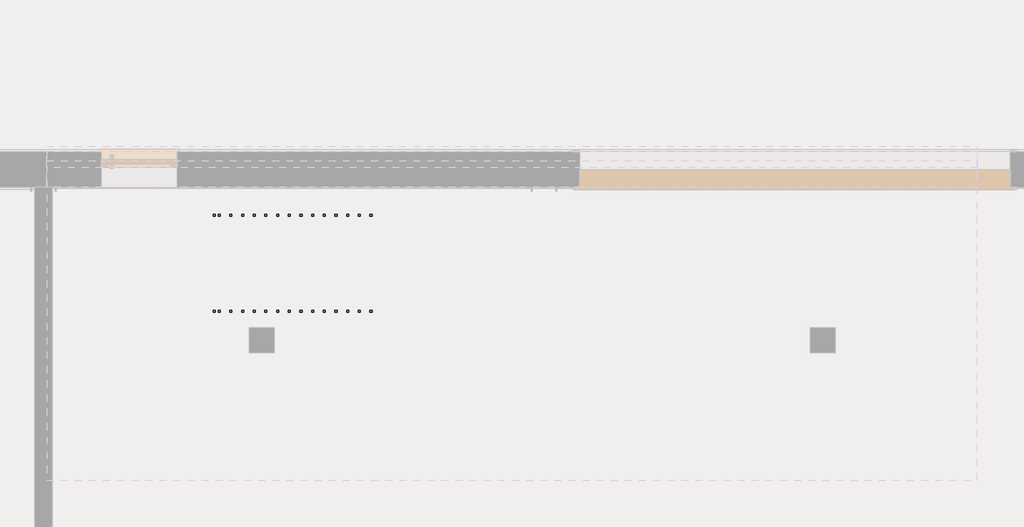
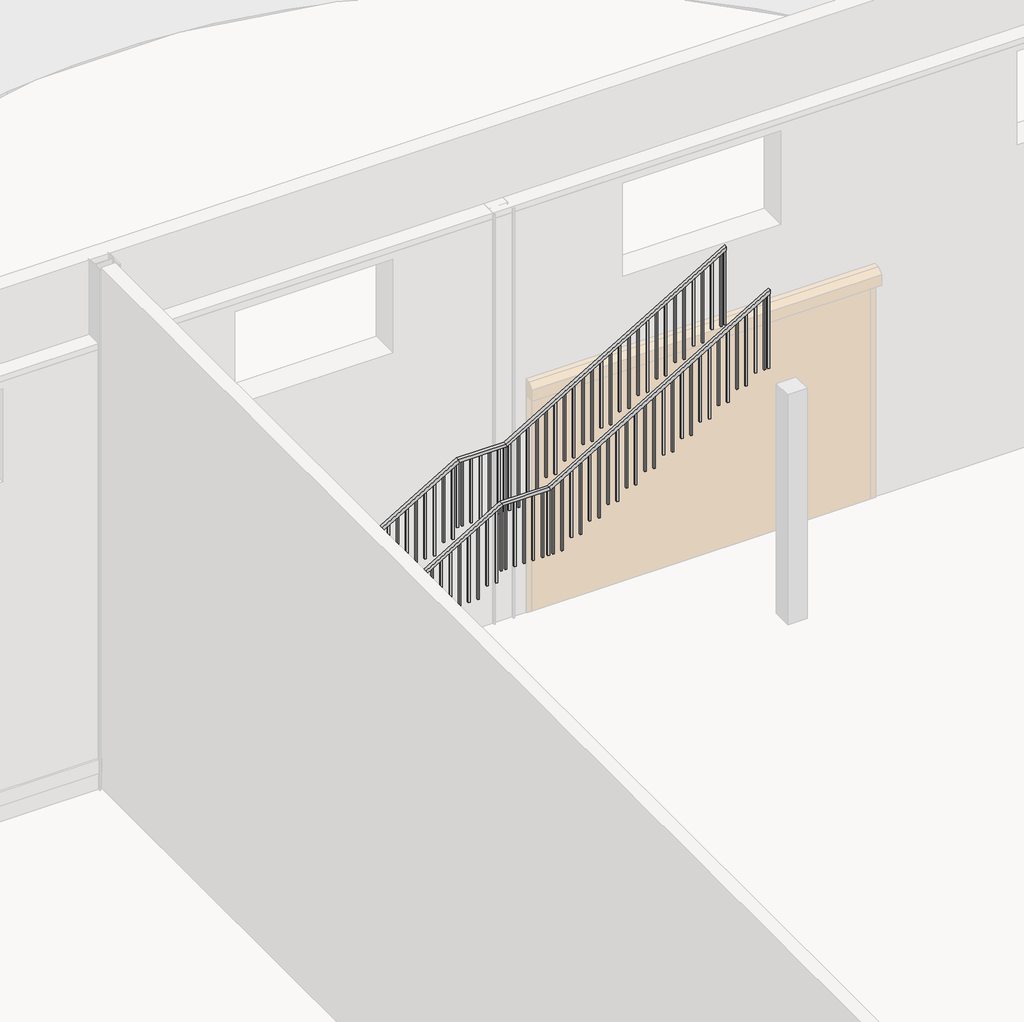
# One storey, part 11 of 13: 2 railings.
"""IFC4 building model written with IfcOpenShell, lengths in millimetres."""

from ifc_helpers import new_model, si_unit, frame, origin, place, context, project, spatial, polyline, outline, extrude, faceted_brep, element, save

model = new_model("IFC4")

# Units and contexts
model_context = context("Model", 3, world=origin())
ifc_project = project(units=[si_unit("LENGTHUNIT", "METRE", prefix="MILLI")], contexts=[model_context])

# Site, building, storey
site = spatial("IfcSite", under=ifc_project)
building = spatial("IfcBuilding", under=site)
storey = spatial("IfcBuildingStorey", under=building, Name="L0 - Ground Floor (Shadows On)", Elevation=0.0)

# Railings
placement = place(None, origin())
element("IfcRailing", 1, ObjectType="1100mm", at=placement, inside=storey, context=model_context, shape_type="SolidModel", body=[
    faceted_brep([(12896.9831159, 5374.1380918, 1266.6666667), (12896.9831159, 5374.1380918, 1208.4792885), (12896.9831159, 5324.1380918, 1208.4792885), (12896.9831159, 5324.1380918, 1266.6666667), (15976.9831159, 5374.1380918, 3100.0), (15990.7379111, 5374.1380918, 3050.0), (15990.7379111, 5324.1380918, 3050.0), (15976.9831159, 5324.1380918, 3100.0), (16696.9831159, 5374.1380918, 3100.0), (16710.7379111, 5374.1380918, 3050.0), (16710.7379111, 5324.1380918, 3050.0), (16696.9831159, 5324.1380918, 3100.0), (20056.9831159, 5374.1380918, 5100.0), (20056.9831159, 5324.1380918, 5100.0), (20056.9831159, 5324.1380918, 5041.8126219), (20056.9831159, 5374.1380918, 5041.8126219)], [[[0, 1, 2, 3]], [[1, 0, 4, 5]], [[2, 1, 5, 6]], [[3, 2, 6, 7]], [[0, 3, 7, 4]], [[5, 4, 8, 9]], [[6, 5, 9, 10]], [[7, 6, 10, 11]], [[4, 7, 11, 8]], [[12, 13, 14, 15]], [[9, 8, 12, 15]], [[10, 9, 15, 14]], [[11, 10, 14, 13]], [[8, 11, 13, 12]]]),
    extrude(outline(polyline([(4992.705479, 19974.4831159), (3833.3333333, 19974.4831159), (3833.3333333, 19999.4831159), (5007.5864314, 19999.4831159), (4992.705479, 19974.4831159)])), frame((0.0, 5336.6380918, 0.0), z_axis=(0.0, 1.0, 0.0), x_axis=(0.0, 0.0, 1.0)), (0.0, 0.0, 1.0), 25.0),
    extrude(outline(polyline([(4909.3721457, 19834.4831159), (3833.3333333, 19834.4831159), (3833.3333333, 19859.4831159), (4924.253098, 19859.4831159), (4909.3721457, 19834.4831159)])), frame((0.0, 5336.6380918, 0.0), z_axis=(0.0, 1.0, 0.0), x_axis=(0.0, 0.0, 1.0)), (0.0, 0.0, 1.0), 25.0),
    extrude(outline(polyline([(4826.0388123, 19694.4831159), (3666.6666667, 19694.4831159), (3666.6666667, 19719.4831159), (4840.9197647, 19719.4831159), (4826.0388123, 19694.4831159)])), frame((0.0, 5336.6380918, 0.0), z_axis=(0.0, 1.0, 0.0), x_axis=(0.0, 0.0, 1.0)), (0.0, 0.0, 1.0), 25.0),
    extrude(outline(polyline([(4742.705479, 19554.4831159), (3666.6666667, 19554.4831159), (3666.6666667, 19579.4831159), (4757.5864314, 19579.4831159), (4742.705479, 19554.4831159)])), frame((0.0, 5336.6380918, 0.0), z_axis=(0.0, 1.0, 0.0), x_axis=(0.0, 0.0, 1.0)), (0.0, 0.0, 1.0), 25.0),
    extrude(outline(polyline([(4659.3721457, 19414.4831159), (3500.0, 19414.4831159), (3500.0, 19439.4831159), (4674.253098, 19439.4831159), (4659.3721457, 19414.4831159)])), frame((0.0, 5336.6380918, 0.0), z_axis=(0.0, 1.0, 0.0), x_axis=(0.0, 0.0, 1.0)), (0.0, 0.0, 1.0), 25.0),
    extrude(outline(polyline([(4576.0388123, 19274.4831159), (3500.0, 19274.4831159), (3500.0, 19299.4831159), (4590.9197647, 19299.4831159), (4576.0388123, 19274.4831159)])), frame((0.0, 5336.6380918, 0.0), z_axis=(0.0, 1.0, 0.0), x_axis=(0.0, 0.0, 1.0)), (0.0, 0.0, 1.0), 25.0),
    extrude(outline(polyline([(4492.705479, 19134.4831159), (3333.3333333, 19134.4831159), (3333.3333333, 19159.4831159), (4507.5864314, 19159.4831159), (4492.705479, 19134.4831159)])), frame((0.0, 5336.6380918, 0.0), z_axis=(0.0, 1.0, 0.0), x_axis=(0.0, 0.0, 1.0)), (0.0, 0.0, 1.0), 25.0),
    extrude(outline(polyline([(4409.3721457, 18994.4831159), (3333.3333333, 18994.4831159), (3333.3333333, 19019.4831159), (4424.253098, 19019.4831159), (4409.3721457, 18994.4831159)])), frame((0.0, 5336.6380918, 0.0), z_axis=(0.0, 1.0, 0.0), x_axis=(0.0, 0.0, 1.0)), (0.0, 0.0, 1.0), 25.0),
    extrude(outline(polyline([(4326.0388123, 18854.4831159), (3166.6666667, 18854.4831159), (3166.6666667, 18879.4831159), (4340.9197647, 18879.4831159), (4326.0388123, 18854.4831159)])), frame((0.0, 5336.6380918, 0.0), z_axis=(0.0, 1.0, 0.0), x_axis=(0.0, 0.0, 1.0)), (0.0, 0.0, 1.0), 25.0),
    extrude(outline(polyline([(4242.705479, 18714.4831159), (3166.6666667, 18714.4831159), (3166.6666667, 18739.4831159), (4257.5864314, 18739.4831159), (4242.705479, 18714.4831159)])), frame((0.0, 5336.6380918, 0.0), z_axis=(0.0, 1.0, 0.0), x_axis=(0.0, 0.0, 1.0)), (0.0, 0.0, 1.0), 25.0),
    extrude(outline(polyline([(4159.3721457, 18574.4831159), (3000.0, 18574.4831159), (3000.0, 18599.4831159), (4174.253098, 18599.4831159), (4159.3721457, 18574.4831159)])), frame((0.0, 5336.6380918, 0.0), z_axis=(0.0, 1.0, 0.0), x_axis=(0.0, 0.0, 1.0)), (0.0, 0.0, 1.0), 25.0),
    extrude(outline(polyline([(4076.0388123, 18434.4831159), (3000.0, 18434.4831159), (3000.0, 18459.4831159), (4090.9197647, 18459.4831159), (4076.0388123, 18434.4831159)])), frame((0.0, 5336.6380918, 0.0), z_axis=(0.0, 1.0, 0.0), x_axis=(0.0, 0.0, 1.0)), (0.0, 0.0, 1.0), 25.0),
    extrude(outline(polyline([(3992.705479, 18294.4831159), (2833.3333333, 18294.4831159), (2833.3333333, 18319.4831159), (4007.5864314, 18319.4831159), (3992.705479, 18294.4831159)])), frame((0.0, 5336.6380918, 0.0), z_axis=(0.0, 1.0, 0.0), x_axis=(0.0, 0.0, 1.0)), (0.0, 0.0, 1.0), 25.0),
    extrude(outline(polyline([(3909.3721457, 18154.4831159), (2833.3333333, 18154.4831159), (2833.3333333, 18179.4831159), (3924.253098, 18179.4831159), (3909.3721457, 18154.4831159)])), frame((0.0, 5336.6380918, 0.0), z_axis=(0.0, 1.0, 0.0), x_axis=(0.0, 0.0, 1.0)), (0.0, 0.0, 1.0), 25.0),
    extrude(outline(polyline([(3826.0388123, 18014.4831159), (2666.6666667, 18014.4831159), (2666.6666667, 18039.4831159), (3840.9197647, 18039.4831159), (3826.0388123, 18014.4831159)])), frame((0.0, 5336.6380918, 0.0), z_axis=(0.0, 1.0, 0.0), x_axis=(0.0, 0.0, 1.0)), (0.0, 0.0, 1.0), 25.0),
    extrude(outline(polyline([(3742.705479, 17874.4831159), (2666.6666667, 17874.4831159), (2666.6666667, 17899.4831159), (3757.5864314, 17899.4831159), (3742.705479, 17874.4831159)])), frame((0.0, 5336.6380918, 0.0), z_axis=(0.0, 1.0, 0.0), x_axis=(0.0, 0.0, 1.0)), (0.0, 0.0, 1.0), 25.0),
    extrude(outline(polyline([(3659.3721457, 17734.4831159), (2500.0, 17734.4831159), (2500.0, 17759.4831159), (3674.253098, 17759.4831159), (3659.3721457, 17734.4831159)])), frame((0.0, 5336.6380918, 0.0), z_axis=(0.0, 1.0, 0.0), x_axis=(0.0, 0.0, 1.0)), (0.0, 0.0, 1.0), 25.0),
    extrude(outline(polyline([(3576.0388123, 17594.4831159), (2500.0, 17594.4831159), (2500.0, 17619.4831159), (3590.9197647, 17619.4831159), (3576.0388123, 17594.4831159)])), frame((0.0, 5336.6380918, 0.0), z_axis=(0.0, 1.0, 0.0), x_axis=(0.0, 0.0, 1.0)), (0.0, 0.0, 1.0), 25.0),
    extrude(outline(polyline([(3492.705479, 17454.4831159), (2333.3333333, 17454.4831159), (2333.3333333, 17479.4831159), (3507.5864314, 17479.4831159), (3492.705479, 17454.4831159)])), frame((0.0, 5336.6380918, 0.0), z_axis=(0.0, 1.0, 0.0), x_axis=(0.0, 0.0, 1.0)), (0.0, 0.0, 1.0), 25.0),
    extrude(outline(polyline([(3409.3721457, 17314.4831159), (2333.3333333, 17314.4831159), (2333.3333333, 17339.4831159), (3424.253098, 17339.4831159), (3409.3721457, 17314.4831159)])), frame((0.0, 5336.6380918, 0.0), z_axis=(0.0, 1.0, 0.0), x_axis=(0.0, 0.0, 1.0)), (0.0, 0.0, 1.0), 25.0),
    extrude(outline(polyline([(3326.0388123, 17174.4831159), (2166.6666667, 17174.4831159), (2166.6666667, 17199.4831159), (3340.9197647, 17199.4831159), (3326.0388123, 17174.4831159)])), frame((0.0, 5336.6380918, 0.0), z_axis=(0.0, 1.0, 0.0), x_axis=(0.0, 0.0, 1.0)), (0.0, 0.0, 1.0), 25.0),
    extrude(outline(polyline([(3242.705479, 17034.4831159), (2166.6666667, 17034.4831159), (2166.6666667, 17059.4831159), (3257.5864314, 17059.4831159), (3242.705479, 17034.4831159)])), frame((0.0, 5336.6380918, 0.0), z_axis=(0.0, 1.0, 0.0), x_axis=(0.0, 0.0, 1.0)), (0.0, 0.0, 1.0), 25.0),
    extrude(outline(polyline([(3159.3721457, 16894.4831159), (2000.0, 16894.4831159), (2000.0, 16919.4831159), (3174.253098, 16919.4831159), (3159.3721457, 16894.4831159)])), frame((0.0, 5336.6380918, 0.0), z_axis=(0.0, 1.0, 0.0), x_axis=(0.0, 0.0, 1.0)), (0.0, 0.0, 1.0), 25.0),
    extrude(outline(polyline([(3076.0388123, 16754.4831159), (2000.0, 16754.4831159), (2000.0, 16779.4831159), (3090.9197647, 16779.4831159), (3076.0388123, 16754.4831159)])), frame((0.0, 5336.6380918, 0.0), z_axis=(0.0, 1.0, 0.0), x_axis=(0.0, 0.0, 1.0)), (0.0, 0.0, 1.0), 25.0),
    extrude(outline(polyline([(16594.4831159, 5336.6380918), (16594.4831159, 5361.6380918), (16619.4831159, 5361.6380918), (16619.4831159, 5336.6380918), (16594.4831159, 5336.6380918)])), frame((0.0, 0.0, 2000.0), z_axis=(0.0, 0.0, 1.0), x_axis=(1.0, 0.0, 0.0)), (0.0, 0.0, 1.0), 1050.0),
    extrude(outline(polyline([(16454.4831159, 5336.6380918), (16454.4831159, 5361.6380918), (16479.4831159, 5361.6380918), (16479.4831159, 5336.6380918), (16454.4831159, 5336.6380918)])), frame((0.0, 0.0, 2000.0), z_axis=(0.0, 0.0, 1.0), x_axis=(1.0, 0.0, 0.0)), (0.0, 0.0, 1.0), 1050.0),
    extrude(outline(polyline([(16314.4831159, 5336.6380918), (16314.4831159, 5361.6380918), (16339.4831159, 5361.6380918), (16339.4831159, 5336.6380918), (16314.4831159, 5336.6380918)])), frame((0.0, 0.0, 2000.0), z_axis=(0.0, 0.0, 1.0), x_axis=(1.0, 0.0, 0.0)), (0.0, 0.0, 1.0), 1050.0),
    extrude(outline(polyline([(16174.4831159, 5336.6380918), (16174.4831159, 5361.6380918), (16199.4831159, 5361.6380918), (16199.4831159, 5336.6380918), (16174.4831159, 5336.6380918)])), frame((0.0, 0.0, 2000.0), z_axis=(0.0, 0.0, 1.0), x_axis=(1.0, 0.0, 0.0)), (0.0, 0.0, 1.0), 1050.0),
    extrude(outline(polyline([(16034.4831159, 5336.6380918), (16034.4831159, 5361.6380918), (16059.4831159, 5361.6380918), (16059.4831159, 5336.6380918), (16034.4831159, 5336.6380918)])), frame((0.0, 0.0, 2000.0), z_axis=(0.0, 0.0, 1.0), x_axis=(1.0, 0.0, 0.0)), (0.0, 0.0, 1.0), 1050.0),
    extrude(outline(polyline([(2992.705479, 15894.4831159), (1833.3333333, 15894.4831159), (1833.3333333, 15919.4831159), (3007.5864314, 15919.4831159), (2992.705479, 15894.4831159)])), frame((0.0, 5336.6380918, 0.0), z_axis=(0.0, 1.0, 0.0), x_axis=(0.0, 0.0, 1.0)), (0.0, 0.0, 1.0), 25.0),
    extrude(outline(polyline([(2909.3721457, 15754.4831159), (1833.3333333, 15754.4831159), (1833.3333333, 15779.4831159), (2924.253098, 15779.4831159), (2909.3721457, 15754.4831159)])), frame((0.0, 5336.6380918, 0.0), z_axis=(0.0, 1.0, 0.0), x_axis=(0.0, 0.0, 1.0)), (0.0, 0.0, 1.0), 25.0),
    extrude(outline(polyline([(2826.0388123, 15614.4831159), (1666.6666667, 15614.4831159), (1666.6666667, 15639.4831159), (2840.9197647, 15639.4831159), (2826.0388123, 15614.4831159)])), frame((0.0, 5336.6380918, 0.0), z_axis=(0.0, 1.0, 0.0), x_axis=(0.0, 0.0, 1.0)), (0.0, 0.0, 1.0), 25.0),
    extrude(outline(polyline([(2742.705479, 15474.4831159), (1666.6666667, 15474.4831159), (1666.6666667, 15499.4831159), (2757.5864314, 15499.4831159), (2742.705479, 15474.4831159)])), frame((0.0, 5336.6380918, 0.0), z_axis=(0.0, 1.0, 0.0), x_axis=(0.0, 0.0, 1.0)), (0.0, 0.0, 1.0), 25.0),
    extrude(outline(polyline([(2659.3721457, 15334.4831159), (1500.0, 15334.4831159), (1500.0, 15359.4831159), (2674.253098, 15359.4831159), (2659.3721457, 15334.4831159)])), frame((0.0, 5336.6380918, 0.0), z_axis=(0.0, 1.0, 0.0), x_axis=(0.0, 0.0, 1.0)), (0.0, 0.0, 1.0), 25.0),
    extrude(outline(polyline([(2576.0388123, 15194.4831159), (1500.0, 15194.4831159), (1500.0, 15219.4831159), (2590.9197647, 15219.4831159), (2576.0388123, 15194.4831159)])), frame((0.0, 5336.6380918, 0.0), z_axis=(0.0, 1.0, 0.0), x_axis=(0.0, 0.0, 1.0)), (0.0, 0.0, 1.0), 25.0),
    extrude(outline(polyline([(2492.705479, 15054.4831159), (1333.3333333, 15054.4831159), (1333.3333333, 15079.4831159), (2507.5864314, 15079.4831159), (2492.705479, 15054.4831159)])), frame((0.0, 5336.6380918, 0.0), z_axis=(0.0, 1.0, 0.0), x_axis=(0.0, 0.0, 1.0)), (0.0, 0.0, 1.0), 25.0),
    extrude(outline(polyline([(2409.3721457, 14914.4831159), (1333.3333333, 14914.4831159), (1333.3333333, 14939.4831159), (2424.253098, 14939.4831159), (2409.3721457, 14914.4831159)])), frame((0.0, 5336.6380918, 0.0), z_axis=(0.0, 1.0, 0.0), x_axis=(0.0, 0.0, 1.0)), (0.0, 0.0, 1.0), 25.0),
    extrude(outline(polyline([(2326.0388123, 14774.4831159), (1166.6666667, 14774.4831159), (1166.6666667, 14799.4831159), (2340.9197647, 14799.4831159), (2326.0388123, 14774.4831159)])), frame((0.0, 5336.6380918, 0.0), z_axis=(0.0, 1.0, 0.0), x_axis=(0.0, 0.0, 1.0)), (0.0, 0.0, 1.0), 25.0),
    extrude(outline(polyline([(2242.705479, 14634.4831159), (1166.6666667, 14634.4831159), (1166.6666667, 14659.4831159), (2257.5864314, 14659.4831159), (2242.705479, 14634.4831159)])), frame((0.0, 5336.6380918, 0.0), z_axis=(0.0, 1.0, 0.0), x_axis=(0.0, 0.0, 1.0)), (0.0, 0.0, 1.0), 25.0),
    extrude(outline(polyline([(2159.3721457, 14494.4831159), (1000.0, 14494.4831159), (1000.0, 14519.4831159), (2174.253098, 14519.4831159), (2159.3721457, 14494.4831159)])), frame((0.0, 5336.6380918, 0.0), z_axis=(0.0, 1.0, 0.0), x_axis=(0.0, 0.0, 1.0)), (0.0, 0.0, 1.0), 25.0),
    extrude(outline(polyline([(2076.0388123, 14354.4831159), (1000.0, 14354.4831159), (1000.0, 14379.4831159), (2090.9197647, 14379.4831159), (2076.0388123, 14354.4831159)])), frame((0.0, 5336.6380918, 0.0), z_axis=(0.0, 1.0, 0.0), x_axis=(0.0, 0.0, 1.0)), (0.0, 0.0, 1.0), 25.0),
    extrude(outline(polyline([(1992.705479, 14214.4831159), (833.3333333, 14214.4831159), (833.3333333, 14239.4831159), (2007.5864314, 14239.4831159), (1992.705479, 14214.4831159)])), frame((0.0, 5336.6380918, 0.0), z_axis=(0.0, 1.0, 0.0), x_axis=(0.0, 0.0, 1.0)), (0.0, 0.0, 1.0), 25.0),
    extrude(outline(polyline([(1909.3721457, 14074.4831159), (833.3333333, 14074.4831159), (833.3333333, 14099.4831159), (1924.253098, 14099.4831159), (1909.3721457, 14074.4831159)])), frame((0.0, 5336.6380918, 0.0), z_axis=(0.0, 1.0, 0.0), x_axis=(0.0, 0.0, 1.0)), (0.0, 0.0, 1.0), 25.0),
    extrude(outline(polyline([(1826.0388123, 13934.4831159), (666.6666667, 13934.4831159), (666.6666667, 13959.4831159), (1840.9197647, 13959.4831159), (1826.0388123, 13934.4831159)])), frame((0.0, 5336.6380918, 0.0), z_axis=(0.0, 1.0, 0.0), x_axis=(0.0, 0.0, 1.0)), (0.0, 0.0, 1.0), 25.0),
    extrude(outline(polyline([(1742.705479, 13794.4831159), (666.6666667, 13794.4831159), (666.6666667, 13819.4831159), (1757.5864314, 13819.4831159), (1742.705479, 13794.4831159)])), frame((0.0, 5336.6380918, 0.0), z_axis=(0.0, 1.0, 0.0), x_axis=(0.0, 0.0, 1.0)), (0.0, 0.0, 1.0), 25.0),
    extrude(outline(polyline([(1659.3721457, 13654.4831159), (500.0, 13654.4831159), (500.0, 13679.4831159), (1674.253098, 13679.4831159), (1659.3721457, 13654.4831159)])), frame((0.0, 5336.6380918, 0.0), z_axis=(0.0, 1.0, 0.0), x_axis=(0.0, 0.0, 1.0)), (0.0, 0.0, 1.0), 25.0),
    extrude(outline(polyline([(1576.0388123, 13514.4831159), (500.0, 13514.4831159), (500.0, 13539.4831159), (1590.9197647, 13539.4831159), (1576.0388123, 13514.4831159)])), frame((0.0, 5336.6380918, 0.0), z_axis=(0.0, 1.0, 0.0), x_axis=(0.0, 0.0, 1.0)), (0.0, 0.0, 1.0), 25.0),
    extrude(outline(polyline([(1492.705479, 13374.4831159), (333.3333333, 13374.4831159), (333.3333333, 13399.4831159), (1507.5864314, 13399.4831159), (1492.705479, 13374.4831159)])), frame((0.0, 5336.6380918, 0.0), z_axis=(0.0, 1.0, 0.0), x_axis=(0.0, 0.0, 1.0)), (0.0, 0.0, 1.0), 25.0),
    extrude(outline(polyline([(1409.3721457, 13234.4831159), (333.3333333, 13234.4831159), (333.3333333, 13259.4831159), (1424.253098, 13259.4831159), (1409.3721457, 13234.4831159)])), frame((0.0, 5336.6380918, 0.0), z_axis=(0.0, 1.0, 0.0), x_axis=(0.0, 0.0, 1.0)), (0.0, 0.0, 1.0), 25.0),
    extrude(outline(polyline([(1326.0388123, 13094.4831159), (166.6666667, 13094.4831159), (166.6666667, 13119.4831159), (1340.9197647, 13119.4831159), (1326.0388123, 13094.4831159)])), frame((0.0, 5336.6380918, 0.0), z_axis=(0.0, 1.0, 0.0), x_axis=(0.0, 0.0, 1.0)), (0.0, 0.0, 1.0), 25.0),
    extrude(outline(polyline([(1242.705479, 12954.4831159), (166.6666667, 12954.4831159), (166.6666667, 12979.4831159), (1257.5864314, 12979.4831159), (1242.705479, 12954.4831159)])), frame((0.0, 5336.6380918, 0.0), z_axis=(0.0, 1.0, 0.0), x_axis=(0.0, 0.0, 1.0)), (0.0, 0.0, 1.0), 25.0),
    extrude(outline(polyline([(16684.4831159, 5336.6380918), (16684.4831159, 5361.6380918), (16709.4831159, 5361.6380918), (16709.4831159, 5336.6380918), (16684.4831159, 5336.6380918)])), frame((0.0, 0.0, 2000.0), z_axis=(0.0, 0.0, 1.0), x_axis=(1.0, 0.0, 0.0)), (0.0, 0.0, 1.0), 1050.0),
    extrude(outline(polyline([(15964.4831159, 5336.6380918), (15964.4831159, 5361.6380918), (15989.4831159, 5361.6380918), (15989.4831159, 5336.6380918), (15964.4831159, 5336.6380918)])), frame((0.0, 0.0, 2000.0), z_axis=(0.0, 0.0, 1.0), x_axis=(1.0, 0.0, 0.0)), (0.0, 0.0, 1.0), 1050.0),
    extrude(outline(polyline([(5026.9316695, 20031.9831159), (3833.3333333, 20031.9831159), (3833.3333333, 20056.9831159), (5041.8126219, 20056.9831159), (5026.9316695, 20031.9831159)])), frame((0.0, 5336.6380918, 0.0), z_axis=(0.0, 1.0, 0.0), x_axis=(0.0, 0.0, 1.0)), (0.0, 0.0, 1.0), 25.0),
    extrude(outline(polyline([(1208.4792885, 12896.9831159), (166.6666667, 12896.9831159), (166.6666667, 12921.9831159), (1223.3602409, 12921.9831159), (1208.4792885, 12896.9831159)])), frame((0.0, 5336.6380918, 0.0), z_axis=(0.0, 1.0, 0.0), x_axis=(0.0, 0.0, 1.0)), (0.0, 0.0, 1.0), 25.0),
])
element("IfcRailing", 2, ObjectType="1100mm", at=placement, inside=storey, context=model_context, shape_type="SolidModel", body=[
    faceted_brep([(12896.9831159, 6523.3380918, 1266.6666667), (12896.9831159, 6523.3380918, 1208.4792885), (12896.9831159, 6473.3380918, 1208.4792885), (12896.9831159, 6473.3380918, 1266.6666667), (15976.9831159, 6523.3380918, 3100.0), (15990.7379111, 6523.3380918, 3050.0), (15990.7379111, 6473.3380918, 3050.0), (15976.9831159, 6473.3380918, 3100.0), (16696.9831159, 6523.3380918, 3100.0), (16710.7379111, 6523.3380918, 3050.0), (16710.7379111, 6473.3380918, 3050.0), (16696.9831159, 6473.3380918, 3100.0), (20056.9831159, 6523.3380918, 5100.0), (20056.9831159, 6473.3380918, 5100.0), (20056.9831159, 6473.3380918, 5041.8126219), (20056.9831159, 6523.3380918, 5041.8126219)], [[[0, 1, 2, 3]], [[1, 0, 4, 5]], [[2, 1, 5, 6]], [[3, 2, 6, 7]], [[0, 3, 7, 4]], [[5, 4, 8, 9]], [[6, 5, 9, 10]], [[7, 6, 10, 11]], [[4, 7, 11, 8]], [[12, 13, 14, 15]], [[9, 8, 12, 15]], [[10, 9, 15, 14]], [[11, 10, 14, 13]], [[8, 11, 13, 12]]]),
    extrude(outline(polyline([(3833.3333333, 19974.4831159), (3833.3333333, 19999.4831159), (5007.5864314, 19999.4831159), (4992.705479, 19974.4831159), (3833.3333333, 19974.4831159)])), frame((0.0, 6485.8380918, 0.0), z_axis=(0.0, 1.0, 0.0), x_axis=(0.0, 0.0, 1.0)), (0.0, 0.0, 1.0), 25.0),
    extrude(outline(polyline([(3833.3333333, 19834.4831159), (3833.3333333, 19859.4831159), (4924.253098, 19859.4831159), (4909.3721457, 19834.4831159), (3833.3333333, 19834.4831159)])), frame((0.0, 6485.8380918, 0.0), z_axis=(0.0, 1.0, 0.0), x_axis=(0.0, 0.0, 1.0)), (0.0, 0.0, 1.0), 25.0),
    extrude(outline(polyline([(3666.6666667, 19694.4831159), (3666.6666667, 19719.4831159), (4840.9197647, 19719.4831159), (4826.0388123, 19694.4831159), (3666.6666667, 19694.4831159)])), frame((0.0, 6485.8380918, 0.0), z_axis=(0.0, 1.0, 0.0), x_axis=(0.0, 0.0, 1.0)), (0.0, 0.0, 1.0), 25.0),
    extrude(outline(polyline([(3666.6666667, 19554.4831159), (3666.6666667, 19579.4831159), (4757.5864314, 19579.4831159), (4742.705479, 19554.4831159), (3666.6666667, 19554.4831159)])), frame((0.0, 6485.8380918, 0.0), z_axis=(0.0, 1.0, 0.0), x_axis=(0.0, 0.0, 1.0)), (0.0, 0.0, 1.0), 25.0),
    extrude(outline(polyline([(3500.0, 19414.4831159), (3500.0, 19439.4831159), (4674.253098, 19439.4831159), (4659.3721457, 19414.4831159), (3500.0, 19414.4831159)])), frame((0.0, 6485.8380918, 0.0), z_axis=(0.0, 1.0, 0.0), x_axis=(0.0, 0.0, 1.0)), (0.0, 0.0, 1.0), 25.0),
    extrude(outline(polyline([(3500.0, 19274.4831159), (3500.0, 19299.4831159), (4590.9197647, 19299.4831159), (4576.0388123, 19274.4831159), (3500.0, 19274.4831159)])), frame((0.0, 6485.8380918, 0.0), z_axis=(0.0, 1.0, 0.0), x_axis=(0.0, 0.0, 1.0)), (0.0, 0.0, 1.0), 25.0),
    extrude(outline(polyline([(3333.3333333, 19134.4831159), (3333.3333333, 19159.4831159), (4507.5864314, 19159.4831159), (4492.705479, 19134.4831159), (3333.3333333, 19134.4831159)])), frame((0.0, 6485.8380918, 0.0), z_axis=(0.0, 1.0, 0.0), x_axis=(0.0, 0.0, 1.0)), (0.0, 0.0, 1.0), 25.0),
    extrude(outline(polyline([(3333.3333333, 18994.4831159), (3333.3333333, 19019.4831159), (4424.253098, 19019.4831159), (4409.3721457, 18994.4831159), (3333.3333333, 18994.4831159)])), frame((0.0, 6485.8380918, 0.0), z_axis=(0.0, 1.0, 0.0), x_axis=(0.0, 0.0, 1.0)), (0.0, 0.0, 1.0), 25.0),
    extrude(outline(polyline([(3166.6666667, 18854.4831159), (3166.6666667, 18879.4831159), (4340.9197647, 18879.4831159), (4326.0388123, 18854.4831159), (3166.6666667, 18854.4831159)])), frame((0.0, 6485.8380918, 0.0), z_axis=(0.0, 1.0, 0.0), x_axis=(0.0, 0.0, 1.0)), (0.0, 0.0, 1.0), 25.0),
    extrude(outline(polyline([(3166.6666667, 18714.4831159), (3166.6666667, 18739.4831159), (4257.5864314, 18739.4831159), (4242.705479, 18714.4831159), (3166.6666667, 18714.4831159)])), frame((0.0, 6485.8380918, 0.0), z_axis=(0.0, 1.0, 0.0), x_axis=(0.0, 0.0, 1.0)), (0.0, 0.0, 1.0), 25.0),
    extrude(outline(polyline([(3000.0, 18574.4831159), (3000.0, 18599.4831159), (4174.253098, 18599.4831159), (4159.3721457, 18574.4831159), (3000.0, 18574.4831159)])), frame((0.0, 6485.8380918, 0.0), z_axis=(0.0, 1.0, 0.0), x_axis=(0.0, 0.0, 1.0)), (0.0, 0.0, 1.0), 25.0),
    extrude(outline(polyline([(3000.0, 18434.4831159), (3000.0, 18459.4831159), (4090.9197647, 18459.4831159), (4076.0388123, 18434.4831159), (3000.0, 18434.4831159)])), frame((0.0, 6485.8380918, 0.0), z_axis=(0.0, 1.0, 0.0), x_axis=(0.0, 0.0, 1.0)), (0.0, 0.0, 1.0), 25.0),
    extrude(outline(polyline([(2833.3333333, 18294.4831159), (2833.3333333, 18319.4831159), (4007.5864314, 18319.4831159), (3992.705479, 18294.4831159), (2833.3333333, 18294.4831159)])), frame((0.0, 6485.8380918, 0.0), z_axis=(0.0, 1.0, 0.0), x_axis=(0.0, 0.0, 1.0)), (0.0, 0.0, 1.0), 25.0),
    extrude(outline(polyline([(2833.3333333, 18154.4831159), (2833.3333333, 18179.4831159), (3924.253098, 18179.4831159), (3909.3721457, 18154.4831159), (2833.3333333, 18154.4831159)])), frame((0.0, 6485.8380918, 0.0), z_axis=(0.0, 1.0, 0.0), x_axis=(0.0, 0.0, 1.0)), (0.0, 0.0, 1.0), 25.0),
    extrude(outline(polyline([(2666.6666667, 18014.4831159), (2666.6666667, 18039.4831159), (3840.9197647, 18039.4831159), (3826.0388123, 18014.4831159), (2666.6666667, 18014.4831159)])), frame((0.0, 6485.8380918, 0.0), z_axis=(0.0, 1.0, 0.0), x_axis=(0.0, 0.0, 1.0)), (0.0, 0.0, 1.0), 25.0),
    extrude(outline(polyline([(2666.6666667, 17874.4831159), (2666.6666667, 17899.4831159), (3757.5864314, 17899.4831159), (3742.705479, 17874.4831159), (2666.6666667, 17874.4831159)])), frame((0.0, 6485.8380918, 0.0), z_axis=(0.0, 1.0, 0.0), x_axis=(0.0, 0.0, 1.0)), (0.0, 0.0, 1.0), 25.0),
    extrude(outline(polyline([(2500.0, 17734.4831159), (2500.0, 17759.4831159), (3674.253098, 17759.4831159), (3659.3721457, 17734.4831159), (2500.0, 17734.4831159)])), frame((0.0, 6485.8380918, 0.0), z_axis=(0.0, 1.0, 0.0), x_axis=(0.0, 0.0, 1.0)), (0.0, 0.0, 1.0), 25.0),
    extrude(outline(polyline([(2500.0, 17594.4831159), (2500.0, 17619.4831159), (3590.9197647, 17619.4831159), (3576.0388123, 17594.4831159), (2500.0, 17594.4831159)])), frame((0.0, 6485.8380918, 0.0), z_axis=(0.0, 1.0, 0.0), x_axis=(0.0, 0.0, 1.0)), (0.0, 0.0, 1.0), 25.0),
    extrude(outline(polyline([(2333.3333333, 17454.4831159), (2333.3333333, 17479.4831159), (3507.5864314, 17479.4831159), (3492.705479, 17454.4831159), (2333.3333333, 17454.4831159)])), frame((0.0, 6485.8380918, 0.0), z_axis=(0.0, 1.0, 0.0), x_axis=(0.0, 0.0, 1.0)), (0.0, 0.0, 1.0), 25.0),
    extrude(outline(polyline([(2333.3333333, 17314.4831159), (2333.3333333, 17339.4831159), (3424.253098, 17339.4831159), (3409.3721457, 17314.4831159), (2333.3333333, 17314.4831159)])), frame((0.0, 6485.8380918, 0.0), z_axis=(0.0, 1.0, 0.0), x_axis=(0.0, 0.0, 1.0)), (0.0, 0.0, 1.0), 25.0),
    extrude(outline(polyline([(2166.6666667, 17174.4831159), (2166.6666667, 17199.4831159), (3340.9197647, 17199.4831159), (3326.0388123, 17174.4831159), (2166.6666667, 17174.4831159)])), frame((0.0, 6485.8380918, 0.0), z_axis=(0.0, 1.0, 0.0), x_axis=(0.0, 0.0, 1.0)), (0.0, 0.0, 1.0), 25.0),
    extrude(outline(polyline([(2166.6666667, 17034.4831159), (2166.6666667, 17059.4831159), (3257.5864314, 17059.4831159), (3242.705479, 17034.4831159), (2166.6666667, 17034.4831159)])), frame((0.0, 6485.8380918, 0.0), z_axis=(0.0, 1.0, 0.0), x_axis=(0.0, 0.0, 1.0)), (0.0, 0.0, 1.0), 25.0),
    extrude(outline(polyline([(2000.0, 16894.4831159), (2000.0, 16919.4831159), (3174.253098, 16919.4831159), (3159.3721457, 16894.4831159), (2000.0, 16894.4831159)])), frame((0.0, 6485.8380918, 0.0), z_axis=(0.0, 1.0, 0.0), x_axis=(0.0, 0.0, 1.0)), (0.0, 0.0, 1.0), 25.0),
    extrude(outline(polyline([(2000.0, 16754.4831159), (2000.0, 16779.4831159), (3090.9197647, 16779.4831159), (3076.0388123, 16754.4831159), (2000.0, 16754.4831159)])), frame((0.0, 6485.8380918, 0.0), z_axis=(0.0, 1.0, 0.0), x_axis=(0.0, 0.0, 1.0)), (0.0, 0.0, 1.0), 25.0),
    extrude(outline(polyline([(16594.4831159, 6510.8380918), (16619.4831159, 6510.8380918), (16619.4831159, 6485.8380918), (16594.4831159, 6485.8380918), (16594.4831159, 6510.8380918)])), frame((0.0, 0.0, 2000.0), z_axis=(0.0, 0.0, 1.0), x_axis=(1.0, 0.0, 0.0)), (0.0, 0.0, 1.0), 1050.0),
    extrude(outline(polyline([(16454.4831159, 6510.8380918), (16479.4831159, 6510.8380918), (16479.4831159, 6485.8380918), (16454.4831159, 6485.8380918), (16454.4831159, 6510.8380918)])), frame((0.0, 0.0, 2000.0), z_axis=(0.0, 0.0, 1.0), x_axis=(1.0, 0.0, 0.0)), (0.0, 0.0, 1.0), 1050.0),
    extrude(outline(polyline([(16314.4831159, 6510.8380918), (16339.4831159, 6510.8380918), (16339.4831159, 6485.8380918), (16314.4831159, 6485.8380918), (16314.4831159, 6510.8380918)])), frame((0.0, 0.0, 2000.0), z_axis=(0.0, 0.0, 1.0), x_axis=(1.0, 0.0, 0.0)), (0.0, 0.0, 1.0), 1050.0),
    extrude(outline(polyline([(16174.4831159, 6510.8380918), (16199.4831159, 6510.8380918), (16199.4831159, 6485.8380918), (16174.4831159, 6485.8380918), (16174.4831159, 6510.8380918)])), frame((0.0, 0.0, 2000.0), z_axis=(0.0, 0.0, 1.0), x_axis=(1.0, 0.0, 0.0)), (0.0, 0.0, 1.0), 1050.0),
    extrude(outline(polyline([(16034.4831159, 6510.8380918), (16059.4831159, 6510.8380918), (16059.4831159, 6485.8380918), (16034.4831159, 6485.8380918), (16034.4831159, 6510.8380918)])), frame((0.0, 0.0, 2000.0), z_axis=(0.0, 0.0, 1.0), x_axis=(1.0, 0.0, 0.0)), (0.0, 0.0, 1.0), 1050.0),
    extrude(outline(polyline([(1833.3333333, 15894.4831159), (1833.3333333, 15919.4831159), (3007.5864314, 15919.4831159), (2992.705479, 15894.4831159), (1833.3333333, 15894.4831159)])), frame((0.0, 6485.8380918, 0.0), z_axis=(0.0, 1.0, 0.0), x_axis=(0.0, 0.0, 1.0)), (0.0, 0.0, 1.0), 25.0),
    extrude(outline(polyline([(1833.3333333, 15754.4831159), (1833.3333333, 15779.4831159), (2924.253098, 15779.4831159), (2909.3721457, 15754.4831159), (1833.3333333, 15754.4831159)])), frame((0.0, 6485.8380918, 0.0), z_axis=(0.0, 1.0, 0.0), x_axis=(0.0, 0.0, 1.0)), (0.0, 0.0, 1.0), 25.0),
    extrude(outline(polyline([(1666.6666667, 15614.4831159), (1666.6666667, 15639.4831159), (2840.9197647, 15639.4831159), (2826.0388123, 15614.4831159), (1666.6666667, 15614.4831159)])), frame((0.0, 6485.8380918, 0.0), z_axis=(0.0, 1.0, 0.0), x_axis=(0.0, 0.0, 1.0)), (0.0, 0.0, 1.0), 25.0),
    extrude(outline(polyline([(1666.6666667, 15474.4831159), (1666.6666667, 15499.4831159), (2757.5864314, 15499.4831159), (2742.705479, 15474.4831159), (1666.6666667, 15474.4831159)])), frame((0.0, 6485.8380918, 0.0), z_axis=(0.0, 1.0, 0.0), x_axis=(0.0, 0.0, 1.0)), (0.0, 0.0, 1.0), 25.0),
    extrude(outline(polyline([(1500.0, 15334.4831159), (1500.0, 15359.4831159), (2674.253098, 15359.4831159), (2659.3721457, 15334.4831159), (1500.0, 15334.4831159)])), frame((0.0, 6485.8380918, 0.0), z_axis=(0.0, 1.0, 0.0), x_axis=(0.0, 0.0, 1.0)), (0.0, 0.0, 1.0), 25.0),
    extrude(outline(polyline([(1500.0, 15194.4831159), (1500.0, 15219.4831159), (2590.9197647, 15219.4831159), (2576.0388123, 15194.4831159), (1500.0, 15194.4831159)])), frame((0.0, 6485.8380918, 0.0), z_axis=(0.0, 1.0, 0.0), x_axis=(0.0, 0.0, 1.0)), (0.0, 0.0, 1.0), 25.0),
    extrude(outline(polyline([(1333.3333333, 15054.4831159), (1333.3333333, 15079.4831159), (2507.5864314, 15079.4831159), (2492.705479, 15054.4831159), (1333.3333333, 15054.4831159)])), frame((0.0, 6485.8380918, 0.0), z_axis=(0.0, 1.0, 0.0), x_axis=(0.0, 0.0, 1.0)), (0.0, 0.0, 1.0), 25.0),
    extrude(outline(polyline([(1333.3333333, 14914.4831159), (1333.3333333, 14939.4831159), (2424.253098, 14939.4831159), (2409.3721457, 14914.4831159), (1333.3333333, 14914.4831159)])), frame((0.0, 6485.8380918, 0.0), z_axis=(0.0, 1.0, 0.0), x_axis=(0.0, 0.0, 1.0)), (0.0, 0.0, 1.0), 25.0),
    extrude(outline(polyline([(1166.6666667, 14774.4831159), (1166.6666667, 14799.4831159), (2340.9197647, 14799.4831159), (2326.0388123, 14774.4831159), (1166.6666667, 14774.4831159)])), frame((0.0, 6485.8380918, 0.0), z_axis=(0.0, 1.0, 0.0), x_axis=(0.0, 0.0, 1.0)), (0.0, 0.0, 1.0), 25.0),
    extrude(outline(polyline([(1166.6666667, 14634.4831159), (1166.6666667, 14659.4831159), (2257.5864314, 14659.4831159), (2242.705479, 14634.4831159), (1166.6666667, 14634.4831159)])), frame((0.0, 6485.8380918, 0.0), z_axis=(0.0, 1.0, 0.0), x_axis=(0.0, 0.0, 1.0)), (0.0, 0.0, 1.0), 25.0),
    extrude(outline(polyline([(1000.0, 14494.4831159), (1000.0, 14519.4831159), (2174.253098, 14519.4831159), (2159.3721457, 14494.4831159), (1000.0, 14494.4831159)])), frame((0.0, 6485.8380918, 0.0), z_axis=(0.0, 1.0, 0.0), x_axis=(0.0, 0.0, 1.0)), (0.0, 0.0, 1.0), 25.0),
    extrude(outline(polyline([(1000.0, 14354.4831159), (1000.0, 14379.4831159), (2090.9197647, 14379.4831159), (2076.0388123, 14354.4831159), (1000.0, 14354.4831159)])), frame((0.0, 6485.8380918, 0.0), z_axis=(0.0, 1.0, 0.0), x_axis=(0.0, 0.0, 1.0)), (0.0, 0.0, 1.0), 25.0),
    extrude(outline(polyline([(833.3333333, 14214.4831159), (833.3333333, 14239.4831159), (2007.5864314, 14239.4831159), (1992.705479, 14214.4831159), (833.3333333, 14214.4831159)])), frame((0.0, 6485.8380918, 0.0), z_axis=(0.0, 1.0, 0.0), x_axis=(0.0, 0.0, 1.0)), (0.0, 0.0, 1.0), 25.0),
    extrude(outline(polyline([(833.3333333, 14074.4831159), (833.3333333, 14099.4831159), (1924.253098, 14099.4831159), (1909.3721457, 14074.4831159), (833.3333333, 14074.4831159)])), frame((0.0, 6485.8380918, 0.0), z_axis=(0.0, 1.0, 0.0), x_axis=(0.0, 0.0, 1.0)), (0.0, 0.0, 1.0), 25.0),
    extrude(outline(polyline([(666.6666667, 13934.4831159), (666.6666667, 13959.4831159), (1840.9197647, 13959.4831159), (1826.0388123, 13934.4831159), (666.6666667, 13934.4831159)])), frame((0.0, 6485.8380918, 0.0), z_axis=(0.0, 1.0, 0.0), x_axis=(0.0, 0.0, 1.0)), (0.0, 0.0, 1.0), 25.0),
    extrude(outline(polyline([(666.6666667, 13794.4831159), (666.6666667, 13819.4831159), (1757.5864314, 13819.4831159), (1742.705479, 13794.4831159), (666.6666667, 13794.4831159)])), frame((0.0, 6485.8380918, 0.0), z_axis=(0.0, 1.0, 0.0), x_axis=(0.0, 0.0, 1.0)), (0.0, 0.0, 1.0), 25.0),
    extrude(outline(polyline([(500.0, 13654.4831159), (500.0, 13679.4831159), (1674.253098, 13679.4831159), (1659.3721457, 13654.4831159), (500.0, 13654.4831159)])), frame((0.0, 6485.8380918, 0.0), z_axis=(0.0, 1.0, 0.0), x_axis=(0.0, 0.0, 1.0)), (0.0, 0.0, 1.0), 25.0),
    extrude(outline(polyline([(500.0, 13514.4831159), (500.0, 13539.4831159), (1590.9197647, 13539.4831159), (1576.0388123, 13514.4831159), (500.0, 13514.4831159)])), frame((0.0, 6485.8380918, 0.0), z_axis=(0.0, 1.0, 0.0), x_axis=(0.0, 0.0, 1.0)), (0.0, 0.0, 1.0), 25.0),
    extrude(outline(polyline([(333.3333333, 13374.4831159), (333.3333333, 13399.4831159), (1507.5864314, 13399.4831159), (1492.705479, 13374.4831159), (333.3333333, 13374.4831159)])), frame((0.0, 6485.8380918, 0.0), z_axis=(0.0, 1.0, 0.0), x_axis=(0.0, 0.0, 1.0)), (0.0, 0.0, 1.0), 25.0),
    extrude(outline(polyline([(333.3333333, 13234.4831159), (333.3333333, 13259.4831159), (1424.253098, 13259.4831159), (1409.3721457, 13234.4831159), (333.3333333, 13234.4831159)])), frame((0.0, 6485.8380918, 0.0), z_axis=(0.0, 1.0, 0.0), x_axis=(0.0, 0.0, 1.0)), (0.0, 0.0, 1.0), 25.0),
    extrude(outline(polyline([(166.6666667, 13094.4831159), (166.6666667, 13119.4831159), (1340.9197647, 13119.4831159), (1326.0388123, 13094.4831159), (166.6666667, 13094.4831159)])), frame((0.0, 6485.8380918, 0.0), z_axis=(0.0, 1.0, 0.0), x_axis=(0.0, 0.0, 1.0)), (0.0, 0.0, 1.0), 25.0),
    extrude(outline(polyline([(166.6666667, 12954.4831159), (166.6666667, 12979.4831159), (1257.5864314, 12979.4831159), (1242.705479, 12954.4831159), (166.6666667, 12954.4831159)])), frame((0.0, 6485.8380918, 0.0), z_axis=(0.0, 1.0, 0.0), x_axis=(0.0, 0.0, 1.0)), (0.0, 0.0, 1.0), 25.0),
    extrude(outline(polyline([(16684.4831159, 6510.8380918), (16709.4831159, 6510.8380918), (16709.4831159, 6485.8380918), (16684.4831159, 6485.8380918), (16684.4831159, 6510.8380918)])), frame((0.0, 0.0, 2000.0), z_axis=(0.0, 0.0, 1.0), x_axis=(1.0, 0.0, 0.0)), (0.0, 0.0, 1.0), 1050.0),
    extrude(outline(polyline([(15964.4831159, 6510.8380918), (15989.4831159, 6510.8380918), (15989.4831159, 6485.8380918), (15964.4831159, 6485.8380918), (15964.4831159, 6510.8380918)])), frame((0.0, 0.0, 2000.0), z_axis=(0.0, 0.0, 1.0), x_axis=(1.0, 0.0, 0.0)), (0.0, 0.0, 1.0), 1050.0),
    extrude(outline(polyline([(3833.3333333, 20031.9831159), (3833.3333333, 20056.9831159), (5041.8126219, 20056.9831159), (5026.9316695, 20031.9831159), (3833.3333333, 20031.9831159)])), frame((0.0, 6485.8380918, 0.0), z_axis=(0.0, 1.0, 0.0), x_axis=(0.0, 0.0, 1.0)), (0.0, 0.0, 1.0), 25.0),
    extrude(outline(polyline([(166.6666667, 12896.9831159), (166.6666667, 12921.9831159), (1223.3602409, 12921.9831159), (1208.4792885, 12896.9831159), (166.6666667, 12896.9831159)])), frame((0.0, 6485.8380918, 0.0), z_axis=(0.0, 1.0, 0.0), x_axis=(0.0, 0.0, 1.0)), (0.0, 0.0, 1.0), 25.0),
])

save(model, "model.ifc")

# Revit data of these elements
# Type "1100mm"
#   built-in parameter 1008612 = 0.019685 (stored number, unit not read)
#   built-in parameter 1008611 = 0.019685 (stored number, unit not read)
#   built-in parameter 1008609 = 0.902231 (stored number, unit not read)
#   built-in parameter 1008604 = 0.19685 (stored number, unit not read)
#   built-in parameter 1008603 = 0.164042 (stored number, unit not read)
#   Railing Height = 1100 mm
#   built-in parameter 1008630 = 2
#   built-in parameter 1008610 = 2
#   built-in parameter 1008608 = 1
#   built-in parameter 1008618 = Baluster - Square : 25mm
# Elements 1, 2 (IfcRailing, "1100mm")
#   Phase Created = New Construction
